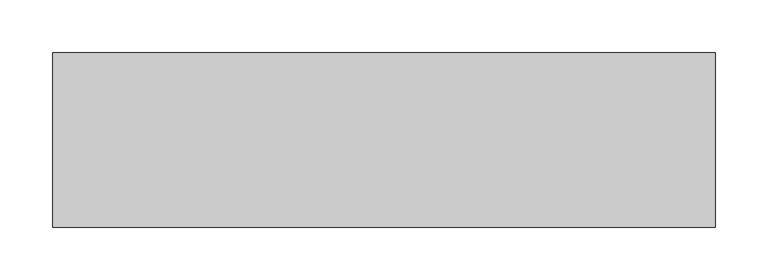
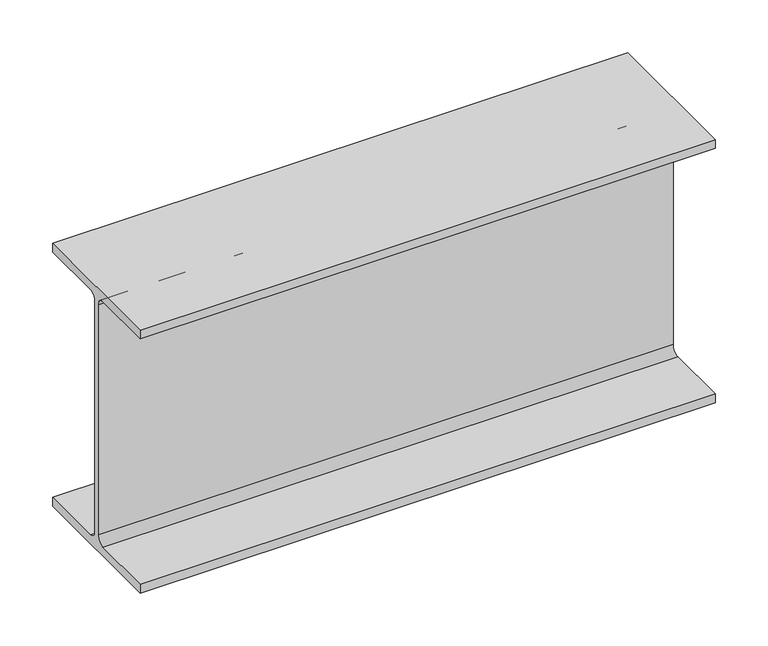
"""IFC4 building model written with IfcOpenShell, lengths in millimetres: beam geometry, Old_Steel Beam_H-KSD3502 : H_SB_ASB_H-300×150x6.5x9."""

from ifc_helpers import new_model, si_unit, point, frame, frame_2d, origin, place, context, project, spatial, polyline, circle_curve, trimmed, segment, composite_curve, outline, extrude, source, transform, mapped, element, save


def beam_8aa6fa65(model_context):
    return source(origin(), model_context, "Body", "SweptSolid", [
        extrude(outline(composite_curve([segment(polyline([(82.5, -141.5), (82.5, -151.7), (-82.5, -151.7), (-82.5, -141.5), (-11.9, -141.5)]), True, "CONTINUOUS"), segment(trimmed(circle_curve(frame_2d((-11.9, -132.6)), 8.9), [point((-11.9, -141.5))], [point((-3.0, -132.6))], True, "CARTESIAN"), True, "CONTINUOUS"), segment(polyline([(-3.0, -132.6), (-3.0, 132.6)]), True, "CONTINUOUS"), segment(trimmed(circle_curve(frame_2d((-11.9, 132.6)), 8.9), [point((-3.0, 132.6))], [point((-11.9, 141.5))], True, "CARTESIAN"), True, "CONTINUOUS"), segment(polyline([(-11.9, 141.5), (-82.5, 141.5), (-82.5, 151.7), (82.5, 151.7), (82.5, 141.5), (11.9, 141.5)]), True, "CONTINUOUS"), segment(trimmed(circle_curve(frame_2d((11.9, 132.6)), 8.9), [point((11.9, 141.5))], [point((3.0, 132.6))], True, "CARTESIAN"), True, "CONTINUOUS"), segment(polyline([(3.0, 132.6), (3.0, -132.6)]), True, "CONTINUOUS"), segment(trimmed(circle_curve(frame_2d((11.9, -132.6)), 8.9), [point((3.0, -132.6))], [point((11.9, -141.5))], True, "CARTESIAN"), True, "CONTINUOUS"), segment(polyline([(11.9, -141.5), (82.5, -141.5)]), True, "CONTINUOUS")], self_intersect=False)), frame((-82.3, 0.0, 0.0), z_axis=(1.0, 0.0, 0.0), x_axis=(0.0, 1.0, 0.0)), (0.0, 0.0, 1.0), 627.3),
    ])


if __name__ == "__main__":
    model = new_model("IFC4")
    model_context = context("Model", 3, world=origin())
    ifc_project = project(units=[si_unit("LENGTHUNIT", "METRE", prefix="MILLI")], contexts=[model_context])
    site = spatial("IfcSite", under=ifc_project)
    building = spatial("IfcBuilding", under=site)
    placement = place(None, origin())
    beam_shape = beam_8aa6fa65(model_context)
    element("IfcBeam", 1, ObjectType="Old_Steel Beam_H-KSD3502 : H_SB_ASB_H-300×150x6.5x9", at=placement, inside=building, context=model_context, shape_type="MappedRepresentation", body=[
        mapped(beam_shape, transform((0.0, 0.0, 0.0), x_axis=(1.0, 0.0, 0.0), y_axis=(0.0, 1.0, 0.0), z_axis=(0.0, 0.0, 1.0))),
    ])
    save(model, "model.ifc")

# Revit data of these elements
# Type "Old_Steel Beam_H-KSD3502 : H_SB_ASB_H-300×150x6.5x9"
#   Width = 15.0 cm
#   Web Thickness = 0.65 cm
#   Web Fillet = 1.3 cm
#   Warping Constant = 107174.0 cm⁶
#   Torsional Moment of Inertia = 9.9539 cm⁴
#   Torsional Modulus = 1.0 cm³
#   Section Area = 46.78 cm²
#   Plastic Modulus weak axis = 105.0 cm³
#   Plastic Modulus strong axis = 542.0 cm³
#   Perimeter = 1.17 m²/m
#   Nominal Weight = 36.70 kgf/m
#   Moment of Inertia weak axis = 508.00 cm⁴
#   Moment of Inertia strong axis = 7210.00 cm⁴
#   Height = 30.0 cm
#   Flange Thickness = 0.9 cm
#   Elastic Modulus weak axis = 67.7 cm³
#   Elastic Modulus strong axis = 481.0 cm³
#   Centroid Vertical = 15.0 cm
#   Centroid Horizontal = 7.5 cm
#   Length [instance default] = 1.5240 m
#   Structural Material [instance default] = Steel, 45-345
#   Assembly Code = ""
# Element 1 (IfcBeam, "Old_Steel Beam_H-KSD3502 : H_SB_ASB_H-300×150x6.5x9")
#   Structural Material = none
# Materials
#   "Steel, 45-345": class "Metal", colour RGB 189 187 185, transparency 0, Description = "Steel 345 MPa", Cost = 0
